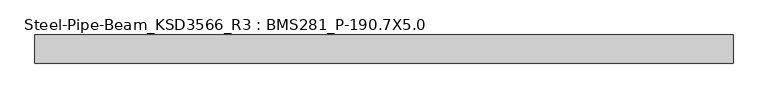
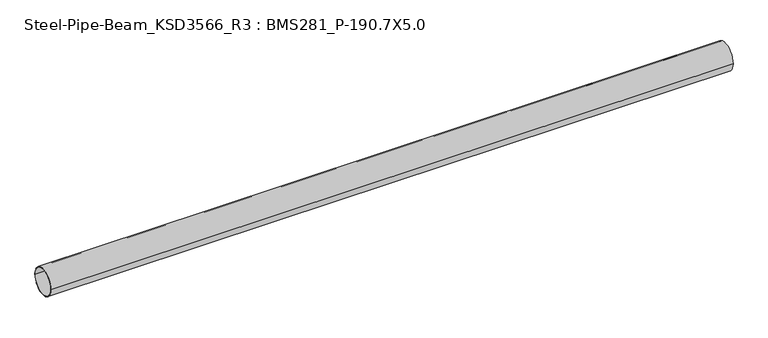
"""IFC4 building model written with IfcOpenShell, lengths in millimetres: member geometry, Steel-Pipe-Beam_KSD3566_R3 : BMS281_P-190.7X5.0."""

from ifc_helpers import new_model, si_unit, point, frame, origin, origin_2d, place, context, project, spatial, circle_curve, trimmed, segment, composite_curve, outline, extrude, source, transform, mapped, element, save


def steel_pipe_beam_ksd3566_r3_bms281_p_190_7x5_0_d9cfb878(model_context):
    return source(origin(), model_context, "Body", "SweptSolid", [
        extrude(outline(composite_curve([segment(trimmed(circle_curve(origin_2d(), 95.35), [point((-95.35, 0.0))], [point((95.35, 0.0))], False, "CARTESIAN"), True, "CONTINUOUS"), segment(trimmed(circle_curve(origin_2d(), 95.35), [point((95.35, 0.0))], [point((-95.35, 0.0))], False, "CARTESIAN"), True, "CONTINUOUS")], self_intersect=False), holes=[composite_curve([segment(trimmed(circle_curve(origin_2d(), 90.35), [point((90.35, 0.0))], [point((-90.35, 0.0))], True, "CARTESIAN"), True, "CONTINUOUS"), segment(trimmed(circle_curve(origin_2d(), 90.35), [point((-90.35, 0.0))], [point((90.35, 0.0))], True, "CARTESIAN"), True, "CONTINUOUS")], self_intersect=False)]), frame((-2315.0256384, 0.0, 0.0), z_axis=(1.0, 0.0, 0.0), x_axis=(0.0, 1.0, 0.0)), (0.0, 0.0, 1.0), 4728.1627144),
    ])


if __name__ == "__main__":
    model = new_model("IFC4")
    model_context = context("Model", 3, world=origin())
    ifc_project = project(units=[si_unit("LENGTHUNIT", "METRE", prefix="MILLI")], contexts=[model_context])
    site = spatial("IfcSite", under=ifc_project)
    building = spatial("IfcBuilding", under=site)
    placement = place(None, origin())
    steel_pipe_beam_ksd3566_r3_bms281_p_190_7x5_0_shape = steel_pipe_beam_ksd3566_r3_bms281_p_190_7x5_0_d9cfb878(model_context)
    element("IfcMember", 1, ObjectType="Steel-Pipe-Beam_KSD3566_R3 : BMS281_P-190.7X5.0", at=placement, inside=building, context=model_context, shape_type="MappedRepresentation", body=[
        mapped(steel_pipe_beam_ksd3566_r3_bms281_p_190_7x5_0_shape, transform((0.0, 0.0, 0.0), x_axis=(1.0, 0.0, 0.0), y_axis=(0.0, 1.0, 0.0), z_axis=(0.0, 0.0, 1.0))),
    ])
    save(model, "model.ifc")

# Revit data of these elements
# Type "Steel-Pipe-Beam_KSD3566_R3 : BMS281_P-190.7X5.0"
#   Keynote = "P-190.7X5.0"
#   SteelWeight = "Light"
#   t = 0.0050 m
#   Surface Area = 0.599102 m²/m
#   Section Area = 29.1697 cm²
#   Mass per Unit Length = 22.8982 kg/m
#   Length [instance default] = 1.5000 m
#   D = 0.1907 m
#   hec_material4 [instance default] = none
#   hec_material3 [instance default] = none
#   hec_material2 [instance default] = none
#   hec_material1 [instance default] = none
#   Structural Material [instance default] = Steel, 45-345
#   Assembly Code = ""
# Element 1 (IfcMember, "Steel-Pipe-Beam_KSD3566_R3 : BMS281_P-190.7X5.0")
#   Structural Material = none
# Materials
#   "Steel, 45-345": class "Metal", colour RGB 189 187 185, transparency 0, Description = "Steel 345 MPa", Cost = 0
